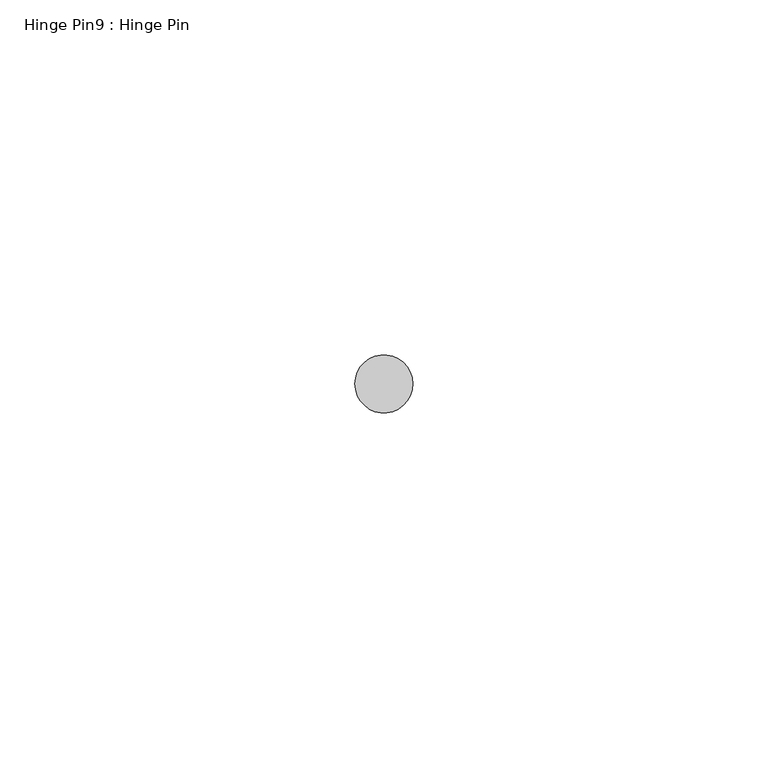
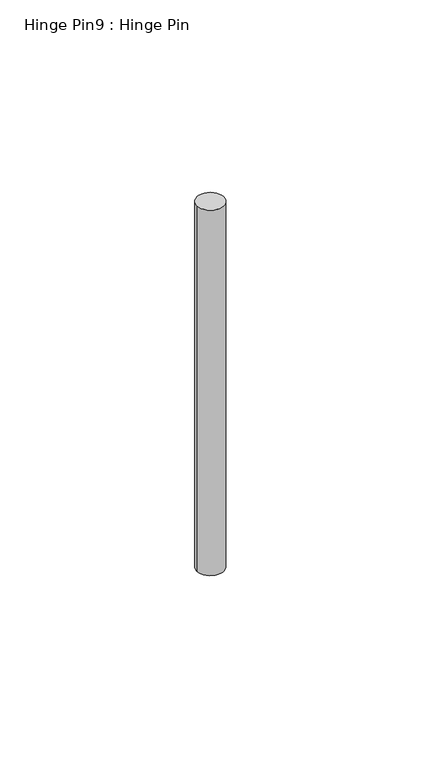
"""IFC4 building model written with IfcOpenShell, lengths in millimetres: proxy geometry, Hinge Pin9 : Hinge Pin."""

from ifc_helpers import new_model, si_unit, point, frame, frame_2d, origin, place, context, project, spatial, circle_curve, trimmed, segment, composite_curve, outline, extrude, source, transform, mapped, element, save


def hinge_pin9_hinge_pin_7a47ebab(model_context):
    return source(origin(), model_context, "Body", "SweptSolid", [
        extrude(outline(composite_curve([segment(trimmed(circle_curve(frame_2d((587319.1320739, -536310.3652841)), 4.0894), [point((587315.0426739, -536310.3652841))], [point((587323.2214739, -536310.3652841))], False, "CARTESIAN"), True, "CONTINUOUS"), segment(trimmed(circle_curve(frame_2d((587319.1320739, -536310.3652841)), 4.0894), [point((587323.2214739, -536310.3652841))], [point((587315.0426739, -536310.3652841))], False, "CARTESIAN"), True, "CONTINUOUS")], self_intersect=False)), frame((0.0, 0.0, 315.7140625), z_axis=(0.0, 0.0, 1.0), x_axis=(1.0, 0.0, 0.0)), (0.0, 0.0, 1.0), 117.871875),
    ])


if __name__ == "__main__":
    model = new_model("IFC4")
    model_context = context("Model", 3, world=origin())
    ifc_project = project(units=[si_unit("LENGTHUNIT", "METRE", prefix="MILLI")], contexts=[model_context])
    site = spatial("IfcSite", under=ifc_project)
    building = spatial("IfcBuilding", under=site)
    placement = place(None, origin())
    hinge_pin9_hinge_pin_shape = hinge_pin9_hinge_pin_7a47ebab(model_context)
    element("IfcBuildingElementProxy", 1, Name="Hinge Pin9 : Hinge Pin", ObjectType="Hinge Pin9 : Hinge Pin", at=placement, inside=building, context=model_context, shape_type="MappedRepresentation", body=[
        mapped(hinge_pin9_hinge_pin_shape, transform((0.0, 0.0, 0.0), x_axis=(1.0, 0.0, 0.0), y_axis=(0.0, 1.0, 0.0), z_axis=(0.0, 0.0, 1.0))),
    ])
    save(model, "model.ifc")

# Revit data of these elements
# Element 1 (IfcBuildingElementProxy, "Hinge Pin9 : Hinge Pin")
#   Materials on its faces: "6\"X6\" WELD-ON STL BUTT HINGE"
# Materials
#   "6\"X6\" WELD-ON STL BUTT HINGE": class "Metal", colour RGB 189 187 185, transparency 0, Description = "Carbon steel", Cost = 0
